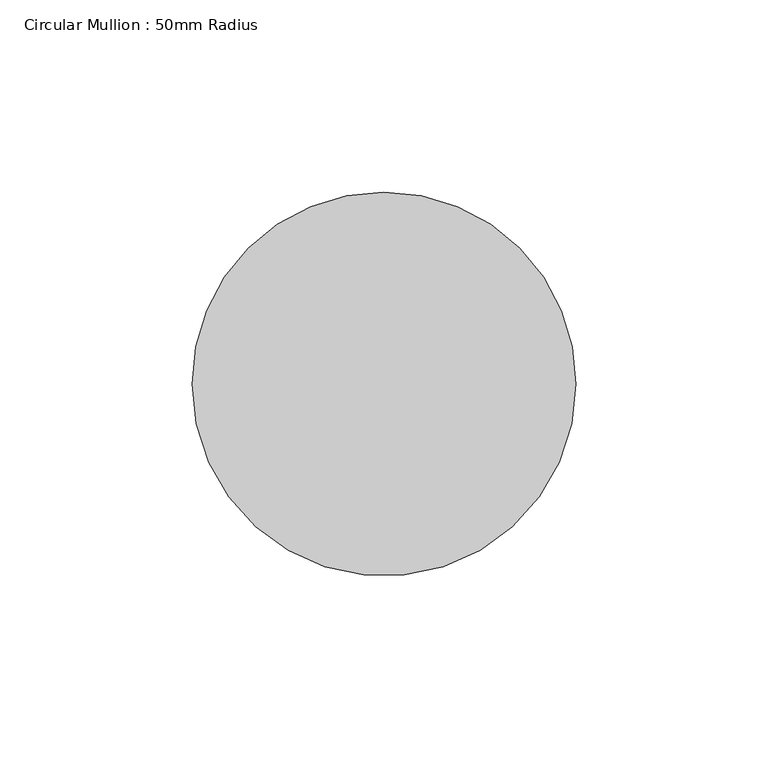
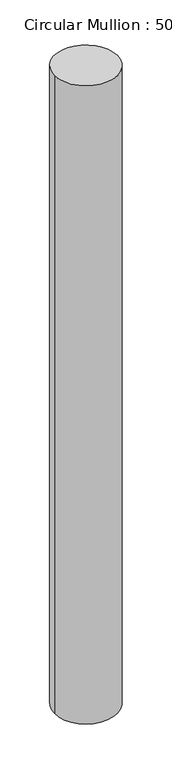
"""IFC4 building model written with IfcOpenShell, lengths in millimetres: member geometry, Circular Mullion : 50mm Radius."""

from ifc_helpers import new_model, si_unit, frame, origin, place, context, project, spatial, ellipse_curve, source, transform, mapped, element, save
from ifc_brep_helpers import plane_surface, cylinder_surface, advanced_brep


def circular_mullion_50mm_radius_0c229c60(model_context):
    return source(origin(), model_context, "Body", "AdvancedBrep", [
        advanced_brep(
        [(-100.0, 0.0, 1.2338829), (0.0, 0.0, 0.0), (0.0, 0.0, -1067.1693152), (-100.0, 0.0, -1068.3639995)],
        [
            (0, 1, ellipse_curve(frame((-50.0, 0.0, 0.6169414), z_axis=(-0.012336512423913957, -0.014940092008921995, -0.9998122844374235), x_axis=(-0.6365992364394205, -0.7709513708897121, 0.019375135819408956)), 50.0093875, 50.0)),
            (1, 2),
            (2, 3, ellipse_curve(frame((-50.0, 0.0, -1067.7666573), z_axis=(-0.011944741256424241, -0.014465638850071733, 0.9998240187397862), x_axis=(0.6366067078898148, 0.770960419164738, 0.018759838779255498)), 50.0088006, 50.0)),
            (3, 0),
            (1, 0, ellipse_curve(frame((-50.0, 0.0, 0.6169414), z_axis=(-0.012336512423913957, -0.014940092008921995, -0.9998122844374235), x_axis=(-0.6365992364394205, -0.7709513708897121, 0.019375135819408956)), 50.0093875, 50.0)),
            (3, 2, ellipse_curve(frame((-50.0, 0.0, -1067.7666573), z_axis=(-0.011944741256424241, -0.014465638850071733, 0.9998240187397862), x_axis=(0.6366067078898148, 0.770960419164738, 0.018759838779255498)), 50.0088006, 50.0)),
        ],
        [
            cylinder_surface(frame((-50.0, 0.0, 0.0), z_axis=(0.0, 0.0, 1.0), x_axis=(1.0, 0.0, 0.0)), 50.0),
            plane_surface(frame((-235.0300967, 194.0718776, 0.0), z_axis=(0.012336512423913957, 0.014940092008921995, 0.9998122844374235), x_axis=(0.6365992364394197, 0.7709513708897127, -0.01937513581940623))),
            plane_surface(frame((-235.0300967, 194.0718776, -1067.1693152), z_axis=(0.011944741256424245, 0.014465638850071736, -0.9998240187397864), x_axis=(0.6366067078898149, 0.770960419164738, 0.01875983877925469))),
        ],
        [
            (0, [[1, 2, 3, 4]]),
            (0, [[5, -4, 6, -2]]),
            (1, [[-1, -5]]),
            (2, [[-6, -3]]),
        ],
    ),
    ])


if __name__ == "__main__":
    model = new_model("IFC4")
    model_context = context("Model", 3, world=origin())
    ifc_project = project(units=[si_unit("LENGTHUNIT", "METRE", prefix="MILLI")], contexts=[model_context])
    site = spatial("IfcSite", under=ifc_project)
    building = spatial("IfcBuilding", under=site)
    placement = place(None, origin())
    circular_mullion_50mm_radius_shape = circular_mullion_50mm_radius_0c229c60(model_context)
    element("IfcMember", 1, ObjectType="Circular Mullion : 50mm Radius", at=placement, inside=building, context=model_context, shape_type="MappedRepresentation", body=[
        mapped(circular_mullion_50mm_radius_shape, transform((0.0, 0.0, 0.0), x_axis=(1.0, 0.0, 0.0), y_axis=(0.0, 1.0, 0.0), z_axis=(0.0, 0.0, 1.0))),
    ])
    save(model, "model.ifc")

# Revit data of these elements
# Type "Circular Mullion : 50mm Radius"
#   built-in parameter 1007350 = 0.164042 (stored number, unit not read)
# Element 1 (IfcMember, "Circular Mullion : 50mm Radius")
#   Materials on its faces: "Aluminium"
# Materials
#   "Aluminium": class "Metal", colour RGB 247 247 247, transparency 0, Description = "Aluminium 6061", Cost = 0
